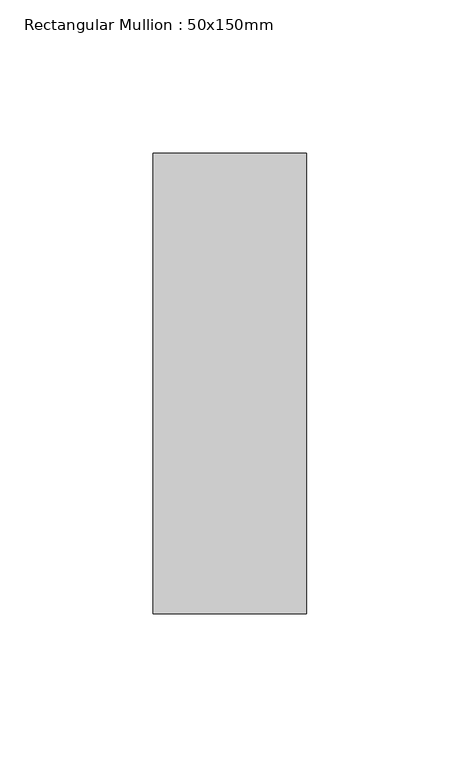
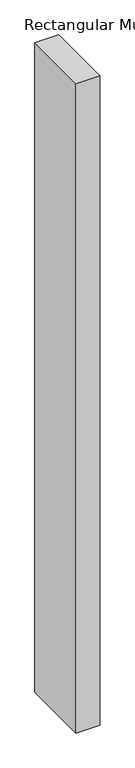
"""IFC4 building model written with IfcOpenShell, lengths in millimetres: member geometry, Rectangular Mullion : 50x150mm."""

from ifc_helpers import new_model, si_unit, frame, origin, place, context, project, spatial, polyline, outline, extrude, source, transform, mapped, element, save


def rectangular_mullion_50x150mm_e3a7335b(model_context):
    return source(origin(), model_context, "Body", "SweptSolid", [
        extrude(outline(polyline([(0.0, 75.0), (0.0, -75.0), (-50.0, -75.0), (-50.0, 75.0), (0.0, 75.0)])), frame((0.0, 0.0, -1449.9999998), z_axis=(0.0, 0.0, 1.0), x_axis=(1.0, 0.0, 0.0)), (0.0, 0.0, 1.0), 1449.9999998),
    ])


if __name__ == "__main__":
    model = new_model("IFC4")
    model_context = context("Model", 3, world=origin())
    ifc_project = project(units=[si_unit("LENGTHUNIT", "METRE", prefix="MILLI")], contexts=[model_context])
    site = spatial("IfcSite", under=ifc_project)
    building = spatial("IfcBuilding", under=site)
    placement = place(None, origin())
    rectangular_mullion_50x150mm_shape = rectangular_mullion_50x150mm_e3a7335b(model_context)
    element("IfcMember", 1, ObjectType="Rectangular Mullion : 50x150mm", at=placement, inside=building, context=model_context, shape_type="MappedRepresentation", body=[
        mapped(rectangular_mullion_50x150mm_shape, transform((0.0, 0.0, 0.0), x_axis=(1.0, 0.0, 0.0), y_axis=(0.0, 1.0, 0.0), z_axis=(0.0, 0.0, 1.0))),
    ])
    save(model, "model.ifc")

# Revit data of these elements
# Type "Rectangular Mullion : 50x150mm"
#   Keynote = "H11"
#   built-in parameter 1007304 = 0.492126 (stored number, unit not read)
#   built-in parameter 1007301 = 0.082021 (stored number, unit not read)
#   built-in parameter 1007300 = 0.082021 (stored number, unit not read)
# Element 1 (IfcMember, "Rectangular Mullion : 50x150mm")
#   Materials on its faces: "Aluminium"
# Materials
#   "Aluminium": class "Metal", colour RGB 247 247 247, transparency 0, Description = "Aluminium 6061", Cost = 0
